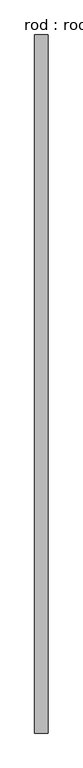
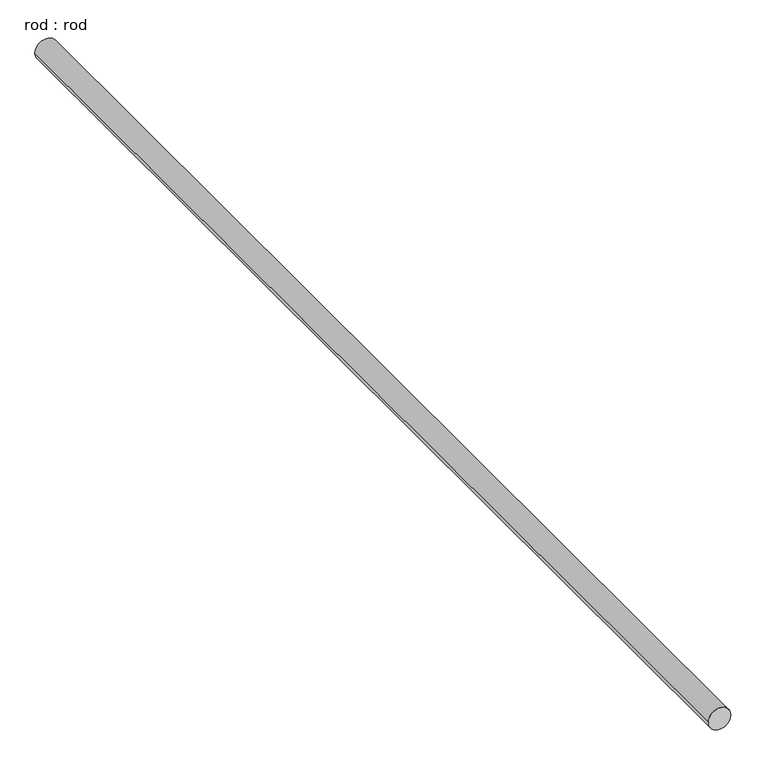
"""IFC4 building model written with IfcOpenShell, lengths in millimetres: proxy geometry, rod : rod."""

from ifc_helpers import new_model, si_unit, point, frame, frame_2d, origin, place, context, project, spatial, circle_curve, trimmed, segment, composite_curve, outline, extrude, source, transform, mapped, element, save


def rod_rod_e0233e5e(model_context):
    return source(origin(), model_context, "Body", "SweptSolid", [
        extrude(outline(composite_curve([segment(trimmed(circle_curve(frame_2d((0.0108462, 0.0)), 200.0), [point((0.0108462, 200.0))], [point((0.0108462, -200.0))], False, "CARTESIAN"), True, "CONTINUOUS"), segment(trimmed(circle_curve(frame_2d((0.0108462, 0.0)), 200.0), [point((0.0108462, -200.0))], [point((0.0108462, 200.0))], False, "CARTESIAN"), True, "CONTINUOUS")], self_intersect=False)), frame((0.0, -6219.3625987, 0.0), z_axis=(0.0, 1.0, 0.0), x_axis=(0.0, 0.0, 1.0)), (0.0, 0.0, 1.0), 20624.1824281),
    ])


if __name__ == "__main__":
    model = new_model("IFC4")
    model_context = context("Model", 3, world=origin())
    ifc_project = project(units=[si_unit("LENGTHUNIT", "METRE", prefix="MILLI")], contexts=[model_context])
    site = spatial("IfcSite", under=ifc_project)
    building = spatial("IfcBuilding", under=site)
    placement = place(None, origin())
    rod_rod_shape = rod_rod_e0233e5e(model_context)
    element("IfcBuildingElementProxy", 1, Name="rod : rod", ObjectType="rod : rod", at=placement, inside=building, context=model_context, shape_type="MappedRepresentation", body=[
        mapped(rod_rod_shape, transform((0.0, 0.0, 0.0), x_axis=(1.0, 0.0, 0.0), y_axis=(0.0, 1.0, 0.0), z_axis=(0.0, 0.0, 1.0))),
    ])
    save(model, "model.ifc")

# Revit data of these elements
# Type "rod : rod"
#   Default Elevation = 0
